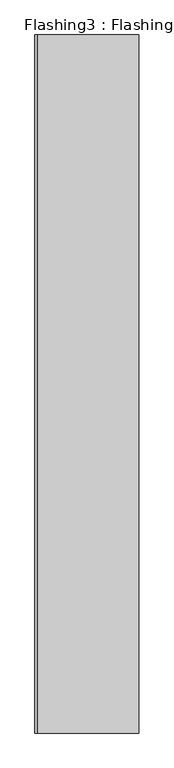
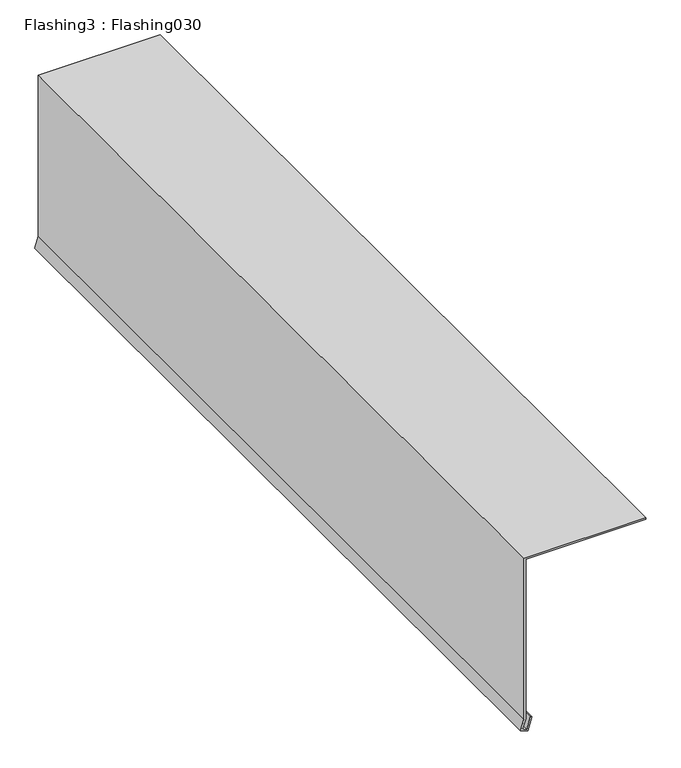
"""IFC4 building model written with IfcOpenShell, lengths in millimetres: proxy geometry, Flashing3 : Flashing030."""

from ifc_helpers import new_model, si_unit, frame, origin, place, context, project, spatial, polyline, outline, extrude, source, transform, mapped, element, save


def flashing3_flashing030_6e34a50e(model_context):
    return source(origin(), model_context, "Body", "SweptSolid", [
        extrude(outline(polyline([(43752.7647284, 5308.7501869), (43725.7732624, 5300.464438), (43720.3821423, 5318.0264272), (43751.7544661, 5327.7395586), (43752.9374956, 5323.9185062), (43725.3718611, 5315.3839573), (43728.4045857, 5305.4564195), (43752.1645952, 5312.7501869), (44153.1848954, 5312.7501869), (44153.1848954, 5598.5706647), (44157.1848954, 5598.5706647), (44157.1848954, 5308.7501869), (43752.7647284, 5308.7501869)])), frame((0.0, -1052.8906574, 0.0), z_axis=(0.0, 1.0, 0.0), x_axis=(0.0, 0.0, 1.0)), (0.0, 0.0, 1.0), 1999.85),
    ])


if __name__ == "__main__":
    model = new_model("IFC4")
    model_context = context("Model", 3, world=origin())
    ifc_project = project(units=[si_unit("LENGTHUNIT", "METRE", prefix="MILLI")], contexts=[model_context])
    site = spatial("IfcSite", under=ifc_project)
    building = spatial("IfcBuilding", under=site)
    placement = place(None, origin())
    flashing3_flashing030_shape = flashing3_flashing030_6e34a50e(model_context)
    element("IfcBuildingElementProxy", 1, Name="Flashing3 : Flashing030", ObjectType="Flashing3 : Flashing030", at=placement, inside=building, context=model_context, shape_type="MappedRepresentation", body=[
        mapped(flashing3_flashing030_shape, transform((0.0, 0.0, 0.0), x_axis=(1.0, 0.0, 0.0), y_axis=(0.0, 1.0, 0.0), z_axis=(0.0, 0.0, 1.0))),
    ])
    save(model, "model.ifc")

# Revit data of these elements
# Type "Flashing3 : Flashing030"
#   NameOverride = "Flashing030"
# Element 1 (IfcBuildingElementProxy, "Flashing3 : Flashing030")
#   Materials on its faces: "BRAKE METAL EAVE TRIM TO MATCH STANDING SEAM COLOR"
# Materials
#   "BRAKE METAL EAVE TRIM TO MATCH STANDING SEAM COLOR": class "Unassigned", colour RGB 128 128 128, transparency 0, Cost = 0
